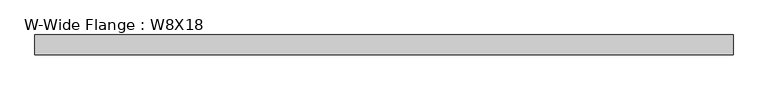
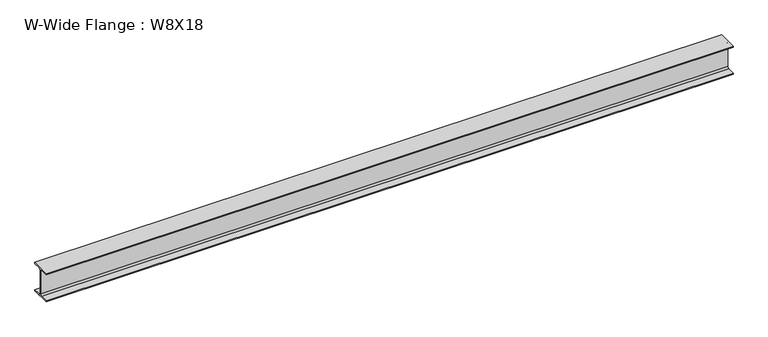
"""IFC4 building model written with IfcOpenShell, lengths in millimetres: beam geometry, W-Wide Flange : W8X18."""

import ifcopenshell
import ifcopenshell.guid

model = None  # the IFC model being written
_history = None  # IfcOwnerHistory: only IFC2X3 demands one
_inside = {}  # id of a spatial element -> (the spatial element, [elements in it])
_under = {}  # id of a project, library or spatial element -> (it, [spatial elements below it])
_declared = {}  # id of a project -> (the project, [libraries it declares])
_typed = {}  # id of a type object -> (the type object, [elements of that type])
_made_of = {}  # id of a material, layer set ... -> (it, [elements and type objects made of it])


def new_model(schema):
    """Start an empty IFC model of exactly this schema.

    Asked for "IFC4X3", IfcOpenShell would pick the latest addendum, in which some entities
    have other attributes; the version numbers below select the first issue.
    IFC2X3 requires an IfcOwnerHistory on every rooted entity: one is made here for all.
    """
    global model, _history
    if schema == "IFC4X3":
        model = ifcopenshell.file(schema_version=(4, 3, 0, 0))
    else:
        model = ifcopenshell.file(schema=schema)
    _inside.clear()
    _under.clear()
    _declared.clear()
    _typed.clear()
    _made_of.clear()
    _history = None
    if model.schema == "IFC2X3":
        org = make("IfcOrganization", Name="unknown")
        user = make(
            "IfcPersonAndOrganization",
            ThePerson=make("IfcPerson", FamilyName="unknown"),
            TheOrganization=org,
        )
        app = make(
            "IfcApplication",
            ApplicationDeveloper=org,
            Version="unknown",
            ApplicationFullName="unknown",
            ApplicationIdentifier="unknown",
        )
        _history = make(
            "IfcOwnerHistory",
            OwningUser=user,
            OwningApplication=app,
            ChangeAction="ADDED",
            CreationDate=0,
        )
    return model


def make(cls, **values):
    """One entity of the class cls with the attributes given. An attribute that is None is left unset."""
    return model.create_entity(
        cls, **{name: value for name, value in values.items() if value is not None}
    )


def rooted(cls, **values):
    """An entity with a GlobalId (a new one), such as an element, a storey or a relation."""
    return make(cls, GlobalId=ifcopenshell.guid.new(), OwnerHistory=_history, **values)


def si_unit(unit_type, name, prefix=None):
    """IfcSIUnit, for example si_unit("LENGTHUNIT", "METRE", prefix="MILLI")."""
    return make("IfcSIUnit", UnitType=unit_type, Prefix=prefix, Name=name)


def assignment(units):
    """IfcUnitAssignment: the units of a project."""
    return None if units is None else make("IfcUnitAssignment", Units=units)


def point(xyz):
    """IfcCartesianPoint."""
    return None if xyz is None else make("IfcCartesianPoint", Coordinates=xyz)


def direction(xyz):
    """IfcDirection."""
    return None if xyz is None else make("IfcDirection", DirectionRatios=xyz)


def frame(location, z_axis=None, x_axis=None):
    """IfcAxis2Placement3D, a coordinate frame: its origin and axes. An axis left out is left unset."""
    return make(
        "IfcAxis2Placement3D",
        Location=point(location),
        Axis=direction(z_axis),
        RefDirection=direction(x_axis),
    )


def frame_2d(location, x_axis=None):
    """IfcAxis2Placement2D, a coordinate frame in the plane: its origin and x axis."""
    return make(
        "IfcAxis2Placement2D", Location=point(location), RefDirection=direction(x_axis)
    )


def origin():
    """The frame at (0, 0, 0) with its axes left unset."""
    return frame((0.0, 0.0, 0.0))


def place(relative_to, where):
    """IfcLocalPlacement: puts the frame where relative to a parent placement (None: the world)."""
    return make(
        "IfcLocalPlacement", PlacementRelTo=relative_to, RelativePlacement=where
    )


def context(
    kind, dimensions, precision=None, world=None, true_north=None, identifier=None
):
    """IfcGeometricRepresentationContext, for example the 3D "Model" context."""
    return make(
        "IfcGeometricRepresentationContext",
        ContextIdentifier=identifier,
        ContextType=kind,
        CoordinateSpaceDimension=dimensions,
        Precision=precision,
        WorldCoordinateSystem=world,
        TrueNorth=true_north,
    )


def project(units=None, contexts=None):
    """IfcProject with its units and contexts."""
    return rooted(
        "IfcProject",
        Name="project",
        RepresentationContexts=contexts,
        UnitsInContext=assignment(units),
    )


def spatial(cls, under=None, at=None, **own):
    """A site, building, storey or space (cls), placed at a placement, below another one or the project."""
    s = rooted(cls, ObjectPlacement=at, **own)
    if under is not None:
        _under.setdefault(under.id(), (under, []))[1].append(s)
    return s


def polyline(points):
    """IfcPolyline through the points."""
    return make("IfcPolyline", Points=[point(p) for p in points])


def circle_curve(where, radius):
    """IfcCircle in the frame where."""
    return make("IfcCircle", Position=where, Radius=radius)


def trimmed(basis, trim1, trim2, sense, master):
    """IfcTrimmedCurve: the piece of a basis curve between two trims."""
    return make(
        "IfcTrimmedCurve",
        BasisCurve=basis,
        Trim1=trim1,
        Trim2=trim2,
        SenseAgreement=sense,
        MasterRepresentation=master,
    )


def segment(curve, same_sense, transition):
    """IfcCompositeCurveSegment."""
    return make(
        "IfcCompositeCurveSegment",
        Transition=transition,
        SameSense=same_sense,
        ParentCurve=curve,
    )


def composite_curve(segments, self_intersect=None):
    """IfcCompositeCurve: segments joined end to end."""
    return make("IfcCompositeCurve", Segments=segments, SelfIntersect=self_intersect)


def outline(outer, holes=None, kind="AREA"):
    """IfcArbitraryClosedProfileDef: a profile drawn as a closed curve; with holes, ...WithVoids."""
    if holes is None:
        return make("IfcArbitraryClosedProfileDef", ProfileType=kind, OuterCurve=outer)
    return make(
        "IfcArbitraryProfileDefWithVoids",
        ProfileType=kind,
        OuterCurve=outer,
        InnerCurves=holes,
    )


def extrude(swept, where, along, depth):
    """IfcExtrudedAreaSolid: the profile swept, set in the frame where, extruded along a direction by depth."""
    return make(
        "IfcExtrudedAreaSolid",
        SweptArea=swept,
        Position=where,
        ExtrudedDirection=direction(along),
        Depth=depth,
    )


def shape(context_of_items, identifier, shape_type, items):
    """IfcShapeRepresentation: the items that make up one representation, for example the "Body"."""
    return make(
        "IfcShapeRepresentation",
        ContextOfItems=context_of_items,
        RepresentationIdentifier=identifier,
        RepresentationType=shape_type,
        Items=items,
    )


def source(mapping_origin, context_of_items, identifier, shape_type, items):
    """IfcRepresentationMap: a shape defined once, which mapped items show again and again."""
    return make(
        "IfcRepresentationMap",
        MappingOrigin=mapping_origin,
        MappedRepresentation=shape(context_of_items, identifier, shape_type, items),
    )


def transform(
    local_origin,
    x_axis=None,
    y_axis=None,
    z_axis=None,
    scale=None,
    scale2=None,
    scale3=None,
    uniform=True,
):
    """IfcCartesianTransformationOperator3D, or its non-uniform kind. x_axis, y_axis, z_axis: its Axis1, 2, 3."""
    if uniform:
        return make(
            "IfcCartesianTransformationOperator3D",
            Axis1=direction(x_axis),
            Axis2=direction(y_axis),
            LocalOrigin=point(local_origin),
            Scale=scale,
            Axis3=direction(z_axis),
        )
    return make(
        "IfcCartesianTransformationOperator3DnonUniform",
        Axis1=direction(x_axis),
        Axis2=direction(y_axis),
        LocalOrigin=point(local_origin),
        Scale=scale,
        Axis3=direction(z_axis),
        Scale2=scale2,
        Scale3=scale3,
    )


def mapped(mapping_source, mapping_target):
    """IfcMappedItem: shows the shape of a source again, moved by a transform."""
    return make(
        "IfcMappedItem", MappingSource=mapping_source, MappingTarget=mapping_target
    )


def made_of(thing, what):
    """Note that an element or type object is made of a material, layer set ...; save() writes the relation."""
    if what is not None:
        _made_of.setdefault(what.id(), (what, []))[1].append(thing)
    return thing


def element(
    cls,
    number,
    at=None,
    inside=None,
    cuts=None,
    type_object=None,
    material=None,
    context=None,
    identifier="Body",
    shape_type=None,
    held_by="IfcProductDefinitionShape",
    body=None,
    shapes=None,
    **own,
):
    """One element of the class cls, such as IfcWall. Its Tag is "e" and its number.

    at: its placement. inside: the storey or other place that contains it. cuts: it is an
    opening in that element (IfcRelVoidsElement). A single representation is given by context,
    identifier, shape_type and body (its items); several are given by shapes. held_by: the class
    of the entity that holds the representations. save() writes the other relations.
    """
    e = rooted(cls, Tag="e%d" % number, ObjectPlacement=at, **own)
    if body is not None:
        shapes = [shape(context, identifier, shape_type, body)]
    if shapes is not None:
        e.Representation = make(held_by, Representations=shapes)
    if inside is not None:
        _inside.setdefault(inside.id(), (inside, []))[1].append(e)
    if cuts is not None:
        rooted(
            "IfcRelVoidsElement", RelatingBuildingElement=cuts, RelatedOpeningElement=e
        )
    if type_object is not None:
        _typed.setdefault(type_object.id(), (type_object, []))[1].append(e)
    return made_of(e, material)


def aggregate(whole, parts):
    """IfcRelAggregates: a whole, such as a stair, and the parts it consists of."""
    return rooted("IfcRelAggregates", RelatingObject=whole, RelatedObjects=parts)


def save(model, path):
    """Write the relations noted so far, then the file.

    IfcRelAggregates (storeys below a building ...), IfcRelContainedInSpatialStructure (elements
    in a storey), IfcRelDefinesByType, IfcRelAssociatesMaterial and IfcRelDeclares: one each for
    every whole, place, type object, material and project.
    """
    for whole, parts in _under.values():
        aggregate(whole, parts)
    for where, things in _inside.values():
        rooted(
            "IfcRelContainedInSpatialStructure",
            RelatedElements=things,
            RelatingStructure=where,
        )
    for kind, things in _typed.values():
        rooted("IfcRelDefinesByType", RelatedObjects=things, RelatingType=kind)
    for what, things in _made_of.values():
        rooted("IfcRelAssociatesMaterial", RelatedObjects=things, RelatingMaterial=what)
    for by, libraries in _declared.values():
        rooted("IfcRelDeclares", RelatingContext=by, RelatedDefinitions=libraries)
    model.write(path)


def w_wide_flange_w8x18_5f46299d(model_context):
    return source(origin(), model_context, "Body", "SweptSolid", [
        extrude(outline(composite_curve([segment(polyline([(66.675, -94.996), (66.675, -103.378), (-66.675, -103.378), (-66.675, -94.996), (-15.1765, -94.996)]), True, "CONTINUOUS"), segment(trimmed(circle_curve(frame_2d((-15.1765, -82.7405)), 12.2555), [point((-15.1765, -94.996))], [point((-2.921, -82.7405))], True, "CARTESIAN"), True, "CONTINUOUS"), segment(polyline([(-2.921, -82.7405), (-2.921, 82.7405)]), True, "CONTINUOUS"), segment(trimmed(circle_curve(frame_2d((-15.1765, 82.7405)), 12.2555), [point((-2.921, 82.7405))], [point((-15.1765, 94.996))], True, "CARTESIAN"), True, "CONTINUOUS"), segment(polyline([(-15.1765, 94.996), (-66.675, 94.996), (-66.675, 103.378), (66.675, 103.378), (66.675, 94.996), (15.1765, 94.996)]), True, "CONTINUOUS"), segment(trimmed(circle_curve(frame_2d((15.1765, 82.7405)), 12.2555), [point((15.1765, 94.996))], [point((2.921, 82.7405))], True, "CARTESIAN"), True, "CONTINUOUS"), segment(polyline([(2.921, 82.7405), (2.921, -82.7405)]), True, "CONTINUOUS"), segment(trimmed(circle_curve(frame_2d((15.1765, -82.7405)), 12.2555), [point((2.921, -82.7405))], [point((15.1765, -94.996))], True, "CARTESIAN"), True, "CONTINUOUS"), segment(polyline([(15.1765, -94.996), (66.675, -94.996)]), True, "CONTINUOUS")], self_intersect=False)), frame((-2388.8051847, 0.0, 0.0), z_axis=(1.0, 0.0, 0.0), x_axis=(0.0, 1.0, 0.0)), (0.0, 0.0, 1.0), 4729.2974575),
    ])


if __name__ == "__main__":
    model = new_model("IFC4")
    model_context = context("Model", 3, world=origin())
    ifc_project = project(units=[si_unit("LENGTHUNIT", "METRE", prefix="MILLI")], contexts=[model_context])
    site = spatial("IfcSite", under=ifc_project)
    building = spatial("IfcBuilding", under=site)
    placement = place(None, origin())
    w_wide_flange_w8x18_shape = w_wide_flange_w8x18_5f46299d(model_context)
    element("IfcBeam", 1, ObjectType="W-Wide Flange : W8X18", at=placement, inside=building, context=model_context, shape_type="MappedRepresentation", body=[
        mapped(w_wide_flange_w8x18_shape, transform((0.0, 0.0, 0.0), x_axis=(1.0, 0.0, 0.0), y_axis=(0.0, 1.0, 0.0), z_axis=(0.0, 0.0, 1.0))),
    ])
    save(model, "model.ifc")

# Revit data of these elements
# Type "W-Wide Flange : W8X18"
#   Assembly Code = "B10"
#   W = 18
#   Length [instance default] = 1524 mm
#   bf = 133.35 mm
#   d = 206.756 mm
#   k = 20.638 mm
#   k2 = 12.256 mm
#   tf = 8.382 mm
#   tw = 5.842 mm
#   A = 0.00339354 m²
#   Structural Material [instance default] = Steel ASTM A992
# Element 1 (IfcBeam, "W-Wide Flange : W8X18")
#   Structural Material = Aluminum, Anodized Red
#   Materials on its faces: "Aluminum, Anodized Red"
# Materials
#   "Steel ASTM A992": class "Metal", colour RGB 128 0 0, transparency 0, Description = "Structural steel 50ksi", Cost = 0
#   "Aluminum, Anodized Red": class "Metal", colour RGB 120 120 120, transparency 0, Description = "Anodized aluminum, red", Cost = 0
